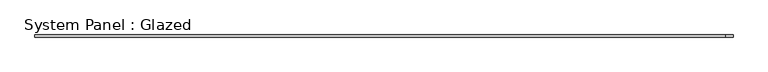
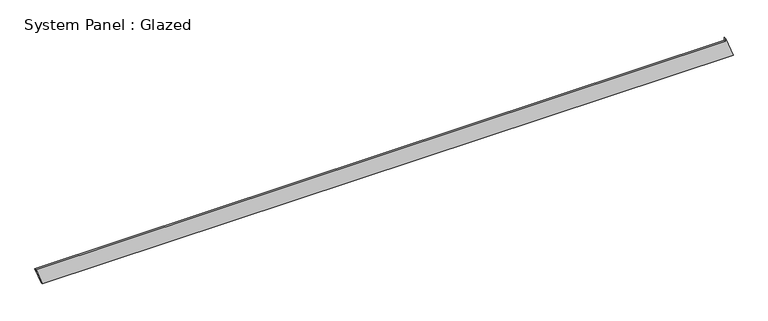
"""IFC4 building model written with IfcOpenShell, lengths in millimetres: plate geometry, System Panel : Glazed."""

import ifcopenshell
import ifcopenshell.guid

model = None  # the IFC model being written
_history = None  # IfcOwnerHistory: only IFC2X3 demands one
_inside = {}  # id of a spatial element -> (the spatial element, [elements in it])
_under = {}  # id of a project, library or spatial element -> (it, [spatial elements below it])
_declared = {}  # id of a project -> (the project, [libraries it declares])
_typed = {}  # id of a type object -> (the type object, [elements of that type])
_made_of = {}  # id of a material, layer set ... -> (it, [elements and type objects made of it])


def new_model(schema):
    """Start an empty IFC model of exactly this schema.

    Asked for "IFC4X3", IfcOpenShell would pick the latest addendum, in which some entities
    have other attributes; the version numbers below select the first issue.
    IFC2X3 requires an IfcOwnerHistory on every rooted entity: one is made here for all.
    """
    global model, _history
    if schema == "IFC4X3":
        model = ifcopenshell.file(schema_version=(4, 3, 0, 0))
    else:
        model = ifcopenshell.file(schema=schema)
    _inside.clear()
    _under.clear()
    _declared.clear()
    _typed.clear()
    _made_of.clear()
    _history = None
    if model.schema == "IFC2X3":
        org = make("IfcOrganization", Name="unknown")
        user = make(
            "IfcPersonAndOrganization",
            ThePerson=make("IfcPerson", FamilyName="unknown"),
            TheOrganization=org,
        )
        app = make(
            "IfcApplication",
            ApplicationDeveloper=org,
            Version="unknown",
            ApplicationFullName="unknown",
            ApplicationIdentifier="unknown",
        )
        _history = make(
            "IfcOwnerHistory",
            OwningUser=user,
            OwningApplication=app,
            ChangeAction="ADDED",
            CreationDate=0,
        )
    return model


def make(cls, **values):
    """One entity of the class cls with the attributes given. An attribute that is None is left unset."""
    return model.create_entity(
        cls, **{name: value for name, value in values.items() if value is not None}
    )


def rooted(cls, **values):
    """An entity with a GlobalId (a new one), such as an element, a storey or a relation."""
    return make(cls, GlobalId=ifcopenshell.guid.new(), OwnerHistory=_history, **values)


def si_unit(unit_type, name, prefix=None):
    """IfcSIUnit, for example si_unit("LENGTHUNIT", "METRE", prefix="MILLI")."""
    return make("IfcSIUnit", UnitType=unit_type, Prefix=prefix, Name=name)


def assignment(units):
    """IfcUnitAssignment: the units of a project."""
    return None if units is None else make("IfcUnitAssignment", Units=units)


def point(xyz):
    """IfcCartesianPoint."""
    return None if xyz is None else make("IfcCartesianPoint", Coordinates=xyz)


def direction(xyz):
    """IfcDirection."""
    return None if xyz is None else make("IfcDirection", DirectionRatios=xyz)


def frame(location, z_axis=None, x_axis=None):
    """IfcAxis2Placement3D, a coordinate frame: its origin and axes. An axis left out is left unset."""
    return make(
        "IfcAxis2Placement3D",
        Location=point(location),
        Axis=direction(z_axis),
        RefDirection=direction(x_axis),
    )


def origin():
    """The frame at (0, 0, 0) with its axes left unset."""
    return frame((0.0, 0.0, 0.0))


def place(relative_to, where):
    """IfcLocalPlacement: puts the frame where relative to a parent placement (None: the world)."""
    return make(
        "IfcLocalPlacement", PlacementRelTo=relative_to, RelativePlacement=where
    )


def context(
    kind, dimensions, precision=None, world=None, true_north=None, identifier=None
):
    """IfcGeometricRepresentationContext, for example the 3D "Model" context."""
    return make(
        "IfcGeometricRepresentationContext",
        ContextIdentifier=identifier,
        ContextType=kind,
        CoordinateSpaceDimension=dimensions,
        Precision=precision,
        WorldCoordinateSystem=world,
        TrueNorth=true_north,
    )


def project(units=None, contexts=None):
    """IfcProject with its units and contexts."""
    return rooted(
        "IfcProject",
        Name="project",
        RepresentationContexts=contexts,
        UnitsInContext=assignment(units),
    )


def spatial(cls, under=None, at=None, **own):
    """A site, building, storey or space (cls), placed at a placement, below another one or the project."""
    s = rooted(cls, ObjectPlacement=at, **own)
    if under is not None:
        _under.setdefault(under.id(), (under, []))[1].append(s)
    return s


def polyline(points):
    """IfcPolyline through the points."""
    return make("IfcPolyline", Points=[point(p) for p in points])


def outline(outer, holes=None, kind="AREA"):
    """IfcArbitraryClosedProfileDef: a profile drawn as a closed curve; with holes, ...WithVoids."""
    if holes is None:
        return make("IfcArbitraryClosedProfileDef", ProfileType=kind, OuterCurve=outer)
    return make(
        "IfcArbitraryProfileDefWithVoids",
        ProfileType=kind,
        OuterCurve=outer,
        InnerCurves=holes,
    )


def extrude(swept, where, along, depth):
    """IfcExtrudedAreaSolid: the profile swept, set in the frame where, extruded along a direction by depth."""
    return make(
        "IfcExtrudedAreaSolid",
        SweptArea=swept,
        Position=where,
        ExtrudedDirection=direction(along),
        Depth=depth,
    )


def shape(context_of_items, identifier, shape_type, items):
    """IfcShapeRepresentation: the items that make up one representation, for example the "Body"."""
    return make(
        "IfcShapeRepresentation",
        ContextOfItems=context_of_items,
        RepresentationIdentifier=identifier,
        RepresentationType=shape_type,
        Items=items,
    )


def source(mapping_origin, context_of_items, identifier, shape_type, items):
    """IfcRepresentationMap: a shape defined once, which mapped items show again and again."""
    return make(
        "IfcRepresentationMap",
        MappingOrigin=mapping_origin,
        MappedRepresentation=shape(context_of_items, identifier, shape_type, items),
    )


def transform(
    local_origin,
    x_axis=None,
    y_axis=None,
    z_axis=None,
    scale=None,
    scale2=None,
    scale3=None,
    uniform=True,
):
    """IfcCartesianTransformationOperator3D, or its non-uniform kind. x_axis, y_axis, z_axis: its Axis1, 2, 3."""
    if uniform:
        return make(
            "IfcCartesianTransformationOperator3D",
            Axis1=direction(x_axis),
            Axis2=direction(y_axis),
            LocalOrigin=point(local_origin),
            Scale=scale,
            Axis3=direction(z_axis),
        )
    return make(
        "IfcCartesianTransformationOperator3DnonUniform",
        Axis1=direction(x_axis),
        Axis2=direction(y_axis),
        LocalOrigin=point(local_origin),
        Scale=scale,
        Axis3=direction(z_axis),
        Scale2=scale2,
        Scale3=scale3,
    )


def mapped(mapping_source, mapping_target):
    """IfcMappedItem: shows the shape of a source again, moved by a transform."""
    return make(
        "IfcMappedItem", MappingSource=mapping_source, MappingTarget=mapping_target
    )


def made_of(thing, what):
    """Note that an element or type object is made of a material, layer set ...; save() writes the relation."""
    if what is not None:
        _made_of.setdefault(what.id(), (what, []))[1].append(thing)
    return thing


def element(
    cls,
    number,
    at=None,
    inside=None,
    cuts=None,
    type_object=None,
    material=None,
    context=None,
    identifier="Body",
    shape_type=None,
    held_by="IfcProductDefinitionShape",
    body=None,
    shapes=None,
    **own,
):
    """One element of the class cls, such as IfcWall. Its Tag is "e" and its number.

    at: its placement. inside: the storey or other place that contains it. cuts: it is an
    opening in that element (IfcRelVoidsElement). A single representation is given by context,
    identifier, shape_type and body (its items); several are given by shapes. held_by: the class
    of the entity that holds the representations. save() writes the other relations.
    """
    e = rooted(cls, Tag="e%d" % number, ObjectPlacement=at, **own)
    if body is not None:
        shapes = [shape(context, identifier, shape_type, body)]
    if shapes is not None:
        e.Representation = make(held_by, Representations=shapes)
    if inside is not None:
        _inside.setdefault(inside.id(), (inside, []))[1].append(e)
    if cuts is not None:
        rooted(
            "IfcRelVoidsElement", RelatingBuildingElement=cuts, RelatedOpeningElement=e
        )
    if type_object is not None:
        _typed.setdefault(type_object.id(), (type_object, []))[1].append(e)
    return made_of(e, material)


def aggregate(whole, parts):
    """IfcRelAggregates: a whole, such as a stair, and the parts it consists of."""
    return rooted("IfcRelAggregates", RelatingObject=whole, RelatedObjects=parts)


def save(model, path):
    """Write the relations noted so far, then the file.

    IfcRelAggregates (storeys below a building ...), IfcRelContainedInSpatialStructure (elements
    in a storey), IfcRelDefinesByType, IfcRelAssociatesMaterial and IfcRelDeclares: one each for
    every whole, place, type object, material and project.
    """
    for whole, parts in _under.values():
        aggregate(whole, parts)
    for where, things in _inside.values():
        rooted(
            "IfcRelContainedInSpatialStructure",
            RelatedElements=things,
            RelatingStructure=where,
        )
    for kind, things in _typed.values():
        rooted("IfcRelDefinesByType", RelatedObjects=things, RelatingType=kind)
    for what, things in _made_of.values():
        rooted("IfcRelAssociatesMaterial", RelatedObjects=things, RelatingMaterial=what)
    for by, libraries in _declared.values():
        rooted("IfcRelDeclares", RelatingContext=by, RelatedDefinitions=libraries)
    model.write(path)


def system_panel_glazed_d7fe694e(model_context):
    return source(origin(), model_context, "Body", "SweptSolid", [
        extrude(outline(polyline([(0.0, -3964.2777152), (0.0, 4035.2773263), (233.2527248, 3950.1929605), (197.8973858, 3950.1906717), (198.4143393, -4035.2773263), (0.0, -3964.2777152)])), frame((0.0, -49.5, 0.0), z_axis=(0.0, 1.0, 0.0), x_axis=(0.0, 0.0, 1.0)), (0.0, 0.0, 1.0), 25.0),
    ])


if __name__ == "__main__":
    model = new_model("IFC4")
    model_context = context("Model", 3, world=origin())
    ifc_project = project(units=[si_unit("LENGTHUNIT", "METRE", prefix="MILLI")], contexts=[model_context])
    site = spatial("IfcSite", under=ifc_project)
    building = spatial("IfcBuilding", under=site)
    placement = place(None, origin())
    system_panel_glazed_shape = system_panel_glazed_d7fe694e(model_context)
    element("IfcPlate", 1, ObjectType="System Panel : Glazed", at=placement, inside=building, context=model_context, shape_type="MappedRepresentation", body=[
        mapped(system_panel_glazed_shape, transform((0.0, 0.0, 0.0), x_axis=(1.0, 0.0, 0.0), y_axis=(0.0, 1.0, 0.0), z_axis=(0.0, 0.0, 1.0))),
    ])
    save(model, "model.ifc")

# Revit data of these elements
# Element 1 (IfcPlate, "System Panel : Glazed")
#   Materials on its faces: "Glass"
# Materials
#   "Glass": class "Glass", colour RGB 218 227 224, transparency 0.85, Description = "Soda Lime Glass", Cost = 0
